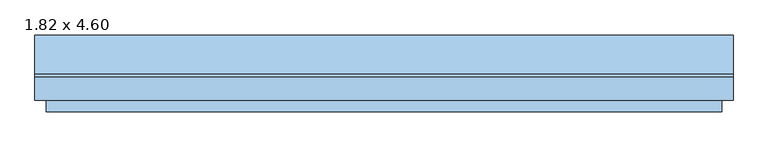
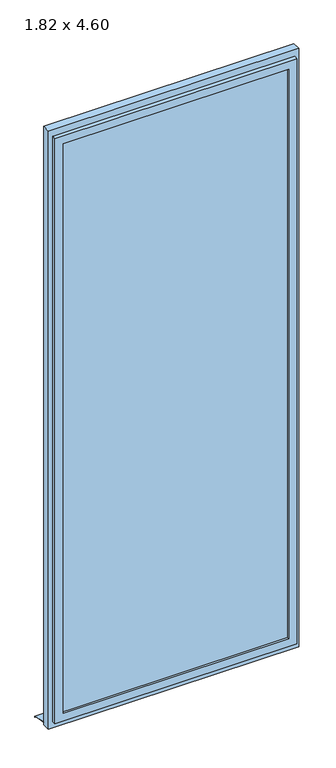
"""IFC4 building model written with IfcOpenShell, lengths in millimetres: window geometry, Fenstertür 1-flg : 1.82 x 4.60."""

import ifcopenshell
import ifcopenshell.guid

model = None  # the IFC model being written
_history = None  # IfcOwnerHistory: only IFC2X3 demands one
_inside = {}  # id of a spatial element -> (the spatial element, [elements in it])
_under = {}  # id of a project, library or spatial element -> (it, [spatial elements below it])
_declared = {}  # id of a project -> (the project, [libraries it declares])
_typed = {}  # id of a type object -> (the type object, [elements of that type])
_made_of = {}  # id of a material, layer set ... -> (it, [elements and type objects made of it])


def new_model(schema):
    """Start an empty IFC model of exactly this schema.

    Asked for "IFC4X3", IfcOpenShell would pick the latest addendum, in which some entities
    have other attributes; the version numbers below select the first issue.
    IFC2X3 requires an IfcOwnerHistory on every rooted entity: one is made here for all.
    """
    global model, _history
    if schema == "IFC4X3":
        model = ifcopenshell.file(schema_version=(4, 3, 0, 0))
    else:
        model = ifcopenshell.file(schema=schema)
    _inside.clear()
    _under.clear()
    _declared.clear()
    _typed.clear()
    _made_of.clear()
    _history = None
    if model.schema == "IFC2X3":
        org = make("IfcOrganization", Name="unknown")
        user = make(
            "IfcPersonAndOrganization",
            ThePerson=make("IfcPerson", FamilyName="unknown"),
            TheOrganization=org,
        )
        app = make(
            "IfcApplication",
            ApplicationDeveloper=org,
            Version="unknown",
            ApplicationFullName="unknown",
            ApplicationIdentifier="unknown",
        )
        _history = make(
            "IfcOwnerHistory",
            OwningUser=user,
            OwningApplication=app,
            ChangeAction="ADDED",
            CreationDate=0,
        )
    return model


def make(cls, **values):
    """One entity of the class cls with the attributes given. An attribute that is None is left unset."""
    return model.create_entity(
        cls, **{name: value for name, value in values.items() if value is not None}
    )


def rooted(cls, **values):
    """An entity with a GlobalId (a new one), such as an element, a storey or a relation."""
    return make(cls, GlobalId=ifcopenshell.guid.new(), OwnerHistory=_history, **values)


def si_unit(unit_type, name, prefix=None):
    """IfcSIUnit, for example si_unit("LENGTHUNIT", "METRE", prefix="MILLI")."""
    return make("IfcSIUnit", UnitType=unit_type, Prefix=prefix, Name=name)


def assignment(units):
    """IfcUnitAssignment: the units of a project."""
    return None if units is None else make("IfcUnitAssignment", Units=units)


def point(xyz):
    """IfcCartesianPoint."""
    return None if xyz is None else make("IfcCartesianPoint", Coordinates=xyz)


def direction(xyz):
    """IfcDirection."""
    return None if xyz is None else make("IfcDirection", DirectionRatios=xyz)


def frame(location, z_axis=None, x_axis=None):
    """IfcAxis2Placement3D, a coordinate frame: its origin and axes. An axis left out is left unset."""
    return make(
        "IfcAxis2Placement3D",
        Location=point(location),
        Axis=direction(z_axis),
        RefDirection=direction(x_axis),
    )


def origin():
    """The frame at (0, 0, 0) with its axes left unset."""
    return frame((0.0, 0.0, 0.0))


def place(relative_to, where):
    """IfcLocalPlacement: puts the frame where relative to a parent placement (None: the world)."""
    return make(
        "IfcLocalPlacement", PlacementRelTo=relative_to, RelativePlacement=where
    )


def context(
    kind, dimensions, precision=None, world=None, true_north=None, identifier=None
):
    """IfcGeometricRepresentationContext, for example the 3D "Model" context."""
    return make(
        "IfcGeometricRepresentationContext",
        ContextIdentifier=identifier,
        ContextType=kind,
        CoordinateSpaceDimension=dimensions,
        Precision=precision,
        WorldCoordinateSystem=world,
        TrueNorth=true_north,
    )


def project(units=None, contexts=None):
    """IfcProject with its units and contexts."""
    return rooted(
        "IfcProject",
        Name="project",
        RepresentationContexts=contexts,
        UnitsInContext=assignment(units),
    )


def spatial(cls, under=None, at=None, **own):
    """A site, building, storey or space (cls), placed at a placement, below another one or the project."""
    s = rooted(cls, ObjectPlacement=at, **own)
    if under is not None:
        _under.setdefault(under.id(), (under, []))[1].append(s)
    return s


def polyline(points):
    """IfcPolyline through the points."""
    return make("IfcPolyline", Points=[point(p) for p in points])


def outline(outer, holes=None, kind="AREA"):
    """IfcArbitraryClosedProfileDef: a profile drawn as a closed curve; with holes, ...WithVoids."""
    if holes is None:
        return make("IfcArbitraryClosedProfileDef", ProfileType=kind, OuterCurve=outer)
    return make(
        "IfcArbitraryProfileDefWithVoids",
        ProfileType=kind,
        OuterCurve=outer,
        InnerCurves=holes,
    )


def extrude(swept, where, along, depth):
    """IfcExtrudedAreaSolid: the profile swept, set in the frame where, extruded along a direction by depth."""
    return make(
        "IfcExtrudedAreaSolid",
        SweptArea=swept,
        Position=where,
        ExtrudedDirection=direction(along),
        Depth=depth,
    )


def faces_of(points, faces, orient=None, outer=None):
    """IfcFace entities. A face is a list of loops; a loop is a list of indices into points, from 0.

    orient and outer hold one flag for each loop. By default every Orientation is true, the
    first loop of a face is its IfcFaceOuterBound and the others are IfcFaceBound.
    """
    made = []
    for i, loops in enumerate(faces):
        bounds = []
        for j, loop in enumerate(loops):
            is_outer = j == 0 if outer is None else outer[i][j]
            bounds.append(
                make(
                    "IfcFaceOuterBound" if is_outer else "IfcFaceBound",
                    Bound=make("IfcPolyLoop", Polygon=[points[k] for k in loop]),
                    Orientation=True if orient is None else orient[i][j],
                )
            )
        made.append(make("IfcFace", Bounds=bounds))
    return made


def faceted_brep(points, faces, orient=None, outer=None, voids=None):
    """IfcFacetedBrep: a solid bounded by flat faces; with voids (closed shells), ...WithVoids."""
    shared = [point(p) for p in points]
    hull = make("IfcClosedShell", CfsFaces=faces_of(shared, faces, orient, outer))
    if voids is None:
        return make("IfcFacetedBrep", Outer=hull)
    return make(
        "IfcFacetedBrepWithVoids",
        Outer=hull,
        Voids=[
            make(cls, CfsFaces=faces_of(shared, fs, o, b)) for cls, fs, o, b in voids
        ],
    )


def shape(context_of_items, identifier, shape_type, items):
    """IfcShapeRepresentation: the items that make up one representation, for example the "Body"."""
    return make(
        "IfcShapeRepresentation",
        ContextOfItems=context_of_items,
        RepresentationIdentifier=identifier,
        RepresentationType=shape_type,
        Items=items,
    )


def source(mapping_origin, context_of_items, identifier, shape_type, items):
    """IfcRepresentationMap: a shape defined once, which mapped items show again and again."""
    return make(
        "IfcRepresentationMap",
        MappingOrigin=mapping_origin,
        MappedRepresentation=shape(context_of_items, identifier, shape_type, items),
    )


def transform(
    local_origin,
    x_axis=None,
    y_axis=None,
    z_axis=None,
    scale=None,
    scale2=None,
    scale3=None,
    uniform=True,
):
    """IfcCartesianTransformationOperator3D, or its non-uniform kind. x_axis, y_axis, z_axis: its Axis1, 2, 3."""
    if uniform:
        return make(
            "IfcCartesianTransformationOperator3D",
            Axis1=direction(x_axis),
            Axis2=direction(y_axis),
            LocalOrigin=point(local_origin),
            Scale=scale,
            Axis3=direction(z_axis),
        )
    return make(
        "IfcCartesianTransformationOperator3DnonUniform",
        Axis1=direction(x_axis),
        Axis2=direction(y_axis),
        LocalOrigin=point(local_origin),
        Scale=scale,
        Axis3=direction(z_axis),
        Scale2=scale2,
        Scale3=scale3,
    )


def mapped(mapping_source, mapping_target):
    """IfcMappedItem: shows the shape of a source again, moved by a transform."""
    return make(
        "IfcMappedItem", MappingSource=mapping_source, MappingTarget=mapping_target
    )


def made_of(thing, what):
    """Note that an element or type object is made of a material, layer set ...; save() writes the relation."""
    if what is not None:
        _made_of.setdefault(what.id(), (what, []))[1].append(thing)
    return thing


def element(
    cls,
    number,
    at=None,
    inside=None,
    cuts=None,
    type_object=None,
    material=None,
    context=None,
    identifier="Body",
    shape_type=None,
    held_by="IfcProductDefinitionShape",
    body=None,
    shapes=None,
    **own,
):
    """One element of the class cls, such as IfcWall. Its Tag is "e" and its number.

    at: its placement. inside: the storey or other place that contains it. cuts: it is an
    opening in that element (IfcRelVoidsElement). A single representation is given by context,
    identifier, shape_type and body (its items); several are given by shapes. held_by: the class
    of the entity that holds the representations. save() writes the other relations.
    """
    e = rooted(cls, Tag="e%d" % number, ObjectPlacement=at, **own)
    if body is not None:
        shapes = [shape(context, identifier, shape_type, body)]
    if shapes is not None:
        e.Representation = make(held_by, Representations=shapes)
    if inside is not None:
        _inside.setdefault(inside.id(), (inside, []))[1].append(e)
    if cuts is not None:
        rooted(
            "IfcRelVoidsElement", RelatingBuildingElement=cuts, RelatedOpeningElement=e
        )
    if type_object is not None:
        _typed.setdefault(type_object.id(), (type_object, []))[1].append(e)
    return made_of(e, material)


def aggregate(whole, parts):
    """IfcRelAggregates: a whole, such as a stair, and the parts it consists of."""
    return rooted("IfcRelAggregates", RelatingObject=whole, RelatedObjects=parts)


def save(model, path):
    """Write the relations noted so far, then the file.

    IfcRelAggregates (storeys below a building ...), IfcRelContainedInSpatialStructure (elements
    in a storey), IfcRelDefinesByType, IfcRelAssociatesMaterial and IfcRelDeclares: one each for
    every whole, place, type object, material and project.
    """
    for whole, parts in _under.values():
        aggregate(whole, parts)
    for where, things in _inside.values():
        rooted(
            "IfcRelContainedInSpatialStructure",
            RelatedElements=things,
            RelatingStructure=where,
        )
    for kind, things in _typed.values():
        rooted("IfcRelDefinesByType", RelatedObjects=things, RelatingType=kind)
    for what, things in _made_of.values():
        rooted("IfcRelAssociatesMaterial", RelatedObjects=things, RelatingMaterial=what)
    for by, libraries in _declared.values():
        rooted("IfcRelDeclares", RelatingContext=by, RelatedDefinitions=libraries)
    model.write(path)


def window_1_82_x_4_60_9a5bc8eb(model_context):
    return source(origin(), model_context, "Body", "SolidModel", [
        extrude(outline(polyline([(4600.0, 910.0), (4600.0, -910.0), (0.0, -910.0), (0.0, 910.0), (4600.0, 910.0)]), holes=[polyline([(4520.0, 850.0), (80.0, 850.0), (80.0, -850.0), (4520.0, -850.0), (4520.0, 850.0)])]), frame((0.0, -80.0, 0.0), z_axis=(0.0, 1.0, 0.0), x_axis=(0.0, 0.0, 1.0)), (0.0, 0.0, 1.0), 60.0),
        faceted_brep([(880.0, -80.0, 4550.0), (880.0, -110.0, 4550.0), (880.0, -110.0, 50.0), (880.0, -80.0, 50.0), (-880.0, -110.0, 4550.0), (-880.0, -110.0, 50.0), (820.0, -110.0, 110.0), (-820.0, -110.0, 110.0), (-820.0, -110.0, 4490.0), (820.0, -110.0, 4490.0), (-880.0, -80.0, 50.0), (-880.0, -80.0, 4550.0), (850.0, -80.0, 4520.0), (-850.0, -80.0, 4520.0), (-850.0, -80.0, 80.0), (850.0, -80.0, 80.0), (850.0, -50.0, 4520.0), (850.0, -50.0, 80.0), (-850.0, -50.0, 80.0), (-850.0, -50.0, 4520.0), (820.0, -50.0, 4490.0), (-820.0, -50.0, 4490.0), (-820.0, -50.0, 110.0), (820.0, -50.0, 110.0)], [[[0, 1, 2, 3]], [[1, 4, 5, 2], [6, 7, 8, 9]], [[3, 2, 5, 10]], [[3, 10, 11, 0], [12, 13, 14, 15]], [[16, 12, 15, 17]], [[17, 15, 14, 18]], [[17, 18, 19, 16], [20, 21, 22, 23]], [[9, 20, 23, 6]], [[6, 23, 22, 7]], [[10, 5, 4, 11]], [[18, 14, 13, 19]], [[7, 22, 21, 8]], [[11, 4, 1, 0]], [[19, 13, 12, 16]], [[8, 21, 20, 9]]]),
        extrude(outline(polyline([(-9.9778457, 20.0), (90.0, 0.0), (90.0, -10.0), (88.0, -10.0), (88.0, -1.6395366), (-10.1759277, 18.0), (-20.0, 18.0), (-20.0, 20.0), (-9.9778457, 20.0)])), frame((-910.0, 0.0, 0.0), z_axis=(1.0, 0.0, 0.0), x_axis=(0.0, 1.0, 0.0)), (0.0, 0.0, 1.0), 1820.0),
        extrude(outline(polyline([(820.0, -95.0), (-820.0, -95.0), (-820.0, -65.0), (820.0, -65.0), (820.0, -95.0)])), frame((0.0, 0.0, 110.0), z_axis=(0.0, 0.0, 1.0), x_axis=(1.0, 0.0, 0.0)), (0.0, 0.0, 1.0), 4380.0),
    ])


if __name__ == "__main__":
    model = new_model("IFC4")
    model_context = context("Model", 3, world=origin())
    ifc_project = project(units=[si_unit("LENGTHUNIT", "METRE", prefix="MILLI")], contexts=[model_context])
    site = spatial("IfcSite", under=ifc_project)
    building = spatial("IfcBuilding", under=site)
    placement = place(None, origin())
    window_1_82_x_4_60_shape = window_1_82_x_4_60_9a5bc8eb(model_context)
    element("IfcWindow", 1, ObjectType="Fenstertür 1-flg : 1.82 x 4.60", at=placement, inside=building, context=model_context, shape_type="MappedRepresentation", body=[
        mapped(window_1_82_x_4_60_shape, transform((0.0, 0.0, 0.0), x_axis=(1.0, 0.0, 0.0), y_axis=(0.0, 1.0, 0.0), z_axis=(0.0, 0.0, 1.0))),
    ])
    save(model, "model.ifc")

# Revit data of these elements
# Type "Fenstertür 1-flg : 1.82 x 4.60"
#   Type Mark = "56"
#   Operation = "SinglePanel"
#   Construction Type Id = "SGL"
#   Keynote = "16.05.01"
#   Analytic Construction = "Große Fenster mit Einfachverglasung"
#   Visual Light Transmittance = 0.9
#   Solar Heat Gain Coefficient = 0.86
#   Rough Width = 1.820 m
#   Rough Height = 4.600 m
#   Heat Transfer Coefficient (U) = 5.5617 W/(m²·K)
#   Rahmentiefe = 0.060 m
#   Rahmenhöhe unten = 0.080 m
#   Höhe oberer  Rahmen = 0.080 m
#   Rahmenbreite = 0.060 m
#   Height = 4.600 m
#   Tiefe Flügel = 0.060 m
#   Flügelbreite = 0.060 m
#   Einbautiefe (von außen) [instance default] = 0.080 m
#   Width = 1.820 m
#   Sichtbarkeit Sturzlinien [instance default] = yes
#   Öffnungsrichtung oben [instance default] = yes
#   Öffnungsrichtung in Draufsicht anzeigen [instance default] = yes
#   Drehflügel 1 [instance default] = yes
#   Bild [instance default] = none
#   Glas [instance default] = none
#   Fensterflügel [instance default] = none
#   Äußere Fensterbank [instance default] = none
#   Wall Closure = (empty or 0)
# Element 1 (IfcWindow, "Fenstertür 1-flg : 1.82 x 4.60")
#   Materials on its faces: "Kunststoff - Weiß", "Glas"
# Materials
#   "Kunststoff - Weiß": class "Kunststoff", colour RGB 249 249 249, transparency 0, Cost = 0
#   "Glas": class "Glas", colour RGB 0 0 255, transparency 0.75, Comments = "Render-Darstellung nicht aktualisiert ", Cost = 0
